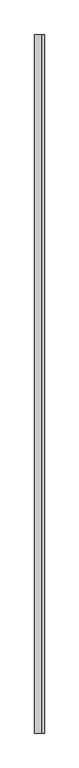
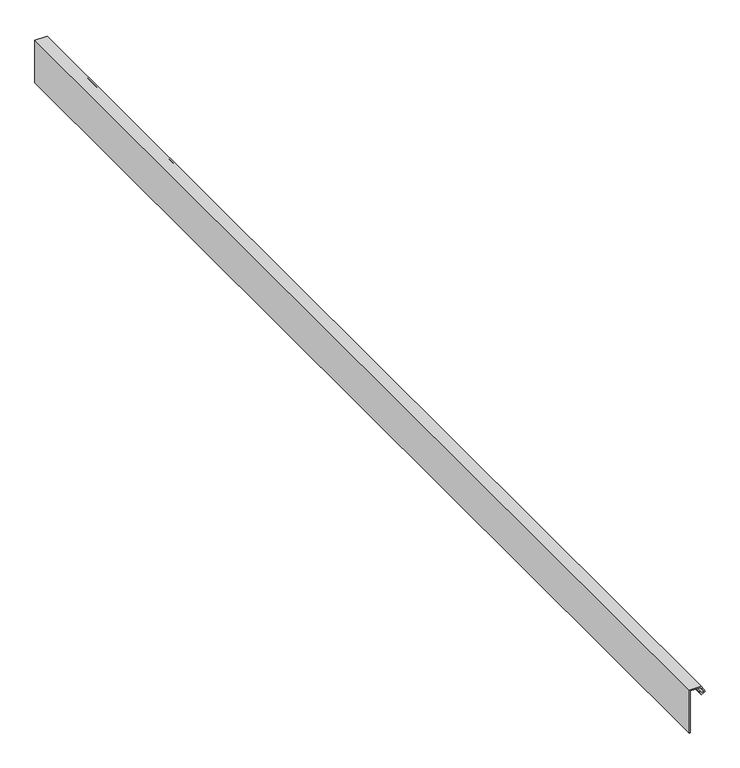
"""IFC4 building model written with IfcOpenShell, lengths in millimetres: proxy geometry, Flashing020 11108 : Flashing020 11108."""

from ifc_helpers import new_model, si_unit, frame, origin, place, context, project, spatial, polyline, outline, extrude, source, transform, mapped, element, save


def generic_models_07dce5c2(model_context):
    return source(origin(), model_context, "Body", "SweptSolid", [
        extrude(outline(polyline([(40707.8367188, 16632.328125), (40785.71875, 16632.328125), (40785.71875, 16650.5221509), (40777.2623654, 16655.298745), (40775.2340727, 16652.1607025), (40779.327926, 16649.9538597), (40778.3789063, 16648.1933594), (40772.3789063, 16651.4277344), (40776.6054688, 16657.9667969), (40787.71875, 16651.6894531), (40787.71875, 16630.328125), (40707.8367188, 16630.328125), (40707.8367188, 16632.328125)])), frame((0.0, 7982.1449112, 0.0), z_axis=(0.0, 1.0, 0.0), x_axis=(0.0, 0.0, 1.0)), (0.0, 0.0, 1.0), 2000.0),
    ])


if __name__ == "__main__":
    model = new_model("IFC4")
    model_context = context("Model", 3, world=origin())
    ifc_project = project(units=[si_unit("LENGTHUNIT", "METRE", prefix="MILLI")], contexts=[model_context])
    site = spatial("IfcSite", under=ifc_project)
    building = spatial("IfcBuilding", under=site)
    placement = place(None, origin())
    generic_models_shape = generic_models_07dce5c2(model_context)
    element("IfcBuildingElementProxy", 1, Name="Flashing020 11108 : Flashing020 11108", ObjectType="Flashing020 11108 : Flashing020 11108", at=placement, inside=building, context=model_context, shape_type="MappedRepresentation", body=[
        mapped(generic_models_shape, transform((0.0, 0.0, 0.0), x_axis=(1.0, 0.0, 0.0), y_axis=(0.0, 1.0, 0.0), z_axis=(0.0, 0.0, 1.0))),
    ])
    save(model, "model.ifc")

# Revit data of these elements
# Type "Flashing020 11108 : Flashing020 11108"
#   NameOverride = "Flashing020"
# Element 1 (IfcBuildingElementProxy, "Flashing020 11108 : Flashing020 11108")
#   Materials on its faces: "BRAKE METAL FLASHING TO MATCH STOREFRONT"
# Materials
#   "BRAKE METAL FLASHING TO MATCH STOREFRONT": class "Unassigned", colour RGB 128 128 128, transparency 0
